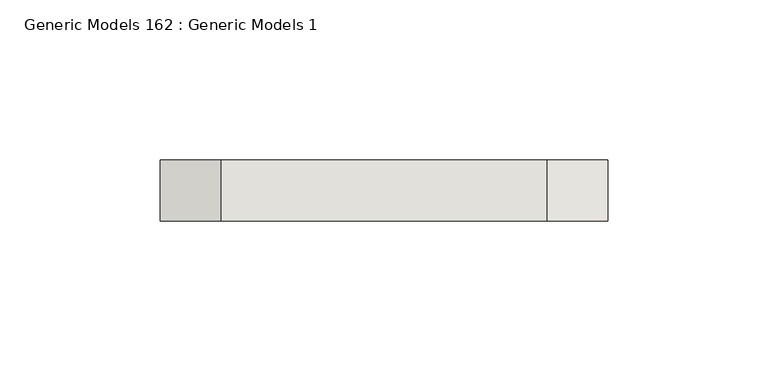
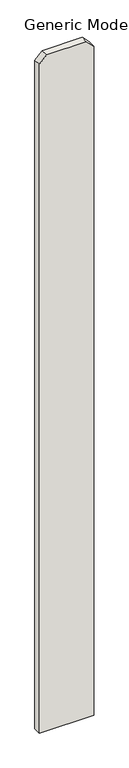
"""IFC4 building model written with IfcOpenShell, lengths in millimetres: wall geometry, Generic Models 162 : Generic Models 1."""

from ifc_helpers import new_model, si_unit, frame, origin, place, context, project, spatial, polyline, outline, extrude, source, transform, mapped, element, save


def generic_models_162_generic_models_1_c4ebdf4a(model_context):
    return source(origin(), model_context, "Body", "SweptSolid", [
        extrude(outline(polyline([(76.2, 323670.6125), (1885.95, 323670.6125), (1905.0, 323651.5625), (1905.0, 323549.9625), (1885.95, 323530.9125), (76.2, 323530.9125), (76.2, 323670.6125)])), frame((0.0, 547.6875, 0.0), z_axis=(0.0, 1.0, 0.0), x_axis=(0.0, 0.0, 1.0)), (0.0, 0.0, 1.0), 19.05),
    ])


if __name__ == "__main__":
    model = new_model("IFC4")
    model_context = context("Model", 3, world=origin())
    ifc_project = project(units=[si_unit("LENGTHUNIT", "METRE", prefix="MILLI")], contexts=[model_context])
    site = spatial("IfcSite", under=ifc_project)
    building = spatial("IfcBuilding", under=site)
    placement = place(None, origin())
    generic_models_162_generic_models_1_shape = generic_models_162_generic_models_1_c4ebdf4a(model_context)
    element("IfcWall", 1, ObjectType="Generic Models 162 : Generic Models 1", at=placement, inside=building, context=model_context, shape_type="MappedRepresentation", body=[
        mapped(generic_models_162_generic_models_1_shape, transform((0.0, 0.0, 0.0), x_axis=(1.0, 0.0, 0.0), y_axis=(0.0, 1.0, 0.0), z_axis=(0.0, 0.0, 1.0))),
    ])
    save(model, "model.ifc")

# Revit data of these elements
# Element 1 (IfcWall, "Generic Models 162 : Generic Models 1")
#   Materials on its faces: "VERTICAL 1X6 CEDAR PLANKS W/ CLEAR WOOD SEALER"
# Materials
#   "VERTICAL 1X6 CEDAR PLANKS W/ CLEAR WOOD SEALER": class "Wood", colour RGB 234 198 147, transparency 0, Description = "Pinus Echinata", Cost = 0
